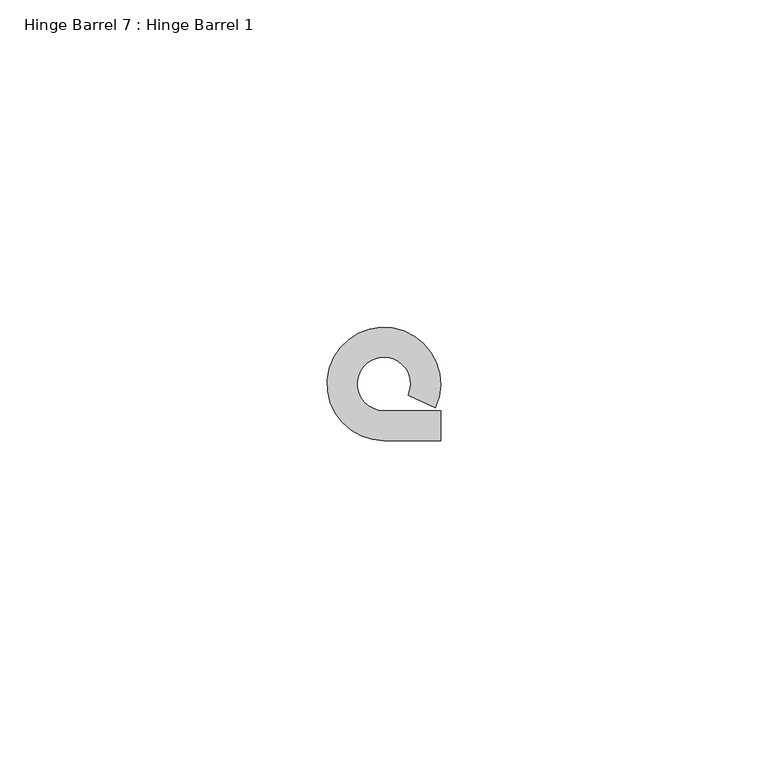
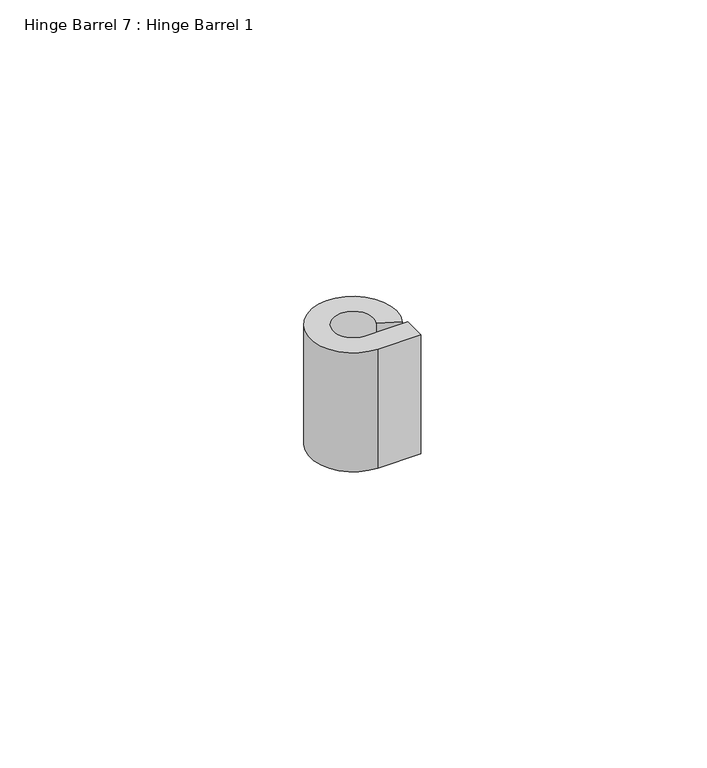
"""IFC4 building model written with IfcOpenShell, lengths in millimetres: proxy geometry, Hinge Barrel 7 : Hinge Barrel 1."""

import ifcopenshell
import ifcopenshell.guid

model = None  # the IFC model being written
_history = None  # IfcOwnerHistory: only IFC2X3 demands one
_inside = {}  # id of a spatial element -> (the spatial element, [elements in it])
_under = {}  # id of a project, library or spatial element -> (it, [spatial elements below it])
_declared = {}  # id of a project -> (the project, [libraries it declares])
_typed = {}  # id of a type object -> (the type object, [elements of that type])
_made_of = {}  # id of a material, layer set ... -> (it, [elements and type objects made of it])


def new_model(schema):
    """Start an empty IFC model of exactly this schema.

    Asked for "IFC4X3", IfcOpenShell would pick the latest addendum, in which some entities
    have other attributes; the version numbers below select the first issue.
    IFC2X3 requires an IfcOwnerHistory on every rooted entity: one is made here for all.
    """
    global model, _history
    if schema == "IFC4X3":
        model = ifcopenshell.file(schema_version=(4, 3, 0, 0))
    else:
        model = ifcopenshell.file(schema=schema)
    _inside.clear()
    _under.clear()
    _declared.clear()
    _typed.clear()
    _made_of.clear()
    _history = None
    if model.schema == "IFC2X3":
        org = make("IfcOrganization", Name="unknown")
        user = make(
            "IfcPersonAndOrganization",
            ThePerson=make("IfcPerson", FamilyName="unknown"),
            TheOrganization=org,
        )
        app = make(
            "IfcApplication",
            ApplicationDeveloper=org,
            Version="unknown",
            ApplicationFullName="unknown",
            ApplicationIdentifier="unknown",
        )
        _history = make(
            "IfcOwnerHistory",
            OwningUser=user,
            OwningApplication=app,
            ChangeAction="ADDED",
            CreationDate=0,
        )
    return model


def make(cls, **values):
    """One entity of the class cls with the attributes given. An attribute that is None is left unset."""
    return model.create_entity(
        cls, **{name: value for name, value in values.items() if value is not None}
    )


def rooted(cls, **values):
    """An entity with a GlobalId (a new one), such as an element, a storey or a relation."""
    return make(cls, GlobalId=ifcopenshell.guid.new(), OwnerHistory=_history, **values)


def si_unit(unit_type, name, prefix=None):
    """IfcSIUnit, for example si_unit("LENGTHUNIT", "METRE", prefix="MILLI")."""
    return make("IfcSIUnit", UnitType=unit_type, Prefix=prefix, Name=name)


def assignment(units):
    """IfcUnitAssignment: the units of a project."""
    return None if units is None else make("IfcUnitAssignment", Units=units)


def point(xyz):
    """IfcCartesianPoint."""
    return None if xyz is None else make("IfcCartesianPoint", Coordinates=xyz)


def direction(xyz):
    """IfcDirection."""
    return None if xyz is None else make("IfcDirection", DirectionRatios=xyz)


def frame(location, z_axis=None, x_axis=None):
    """IfcAxis2Placement3D, a coordinate frame: its origin and axes. An axis left out is left unset."""
    return make(
        "IfcAxis2Placement3D",
        Location=point(location),
        Axis=direction(z_axis),
        RefDirection=direction(x_axis),
    )


def frame_2d(location, x_axis=None):
    """IfcAxis2Placement2D, a coordinate frame in the plane: its origin and x axis."""
    return make(
        "IfcAxis2Placement2D", Location=point(location), RefDirection=direction(x_axis)
    )


def origin():
    """The frame at (0, 0, 0) with its axes left unset."""
    return frame((0.0, 0.0, 0.0))


def place(relative_to, where):
    """IfcLocalPlacement: puts the frame where relative to a parent placement (None: the world)."""
    return make(
        "IfcLocalPlacement", PlacementRelTo=relative_to, RelativePlacement=where
    )


def context(
    kind, dimensions, precision=None, world=None, true_north=None, identifier=None
):
    """IfcGeometricRepresentationContext, for example the 3D "Model" context."""
    return make(
        "IfcGeometricRepresentationContext",
        ContextIdentifier=identifier,
        ContextType=kind,
        CoordinateSpaceDimension=dimensions,
        Precision=precision,
        WorldCoordinateSystem=world,
        TrueNorth=true_north,
    )


def project(units=None, contexts=None):
    """IfcProject with its units and contexts."""
    return rooted(
        "IfcProject",
        Name="project",
        RepresentationContexts=contexts,
        UnitsInContext=assignment(units),
    )


def spatial(cls, under=None, at=None, **own):
    """A site, building, storey or space (cls), placed at a placement, below another one or the project."""
    s = rooted(cls, ObjectPlacement=at, **own)
    if under is not None:
        _under.setdefault(under.id(), (under, []))[1].append(s)
    return s


def polyline(points):
    """IfcPolyline through the points."""
    return make("IfcPolyline", Points=[point(p) for p in points])


def circle_curve(where, radius):
    """IfcCircle in the frame where."""
    return make("IfcCircle", Position=where, Radius=radius)


def trimmed(basis, trim1, trim2, sense, master):
    """IfcTrimmedCurve: the piece of a basis curve between two trims."""
    return make(
        "IfcTrimmedCurve",
        BasisCurve=basis,
        Trim1=trim1,
        Trim2=trim2,
        SenseAgreement=sense,
        MasterRepresentation=master,
    )


def segment(curve, same_sense, transition):
    """IfcCompositeCurveSegment."""
    return make(
        "IfcCompositeCurveSegment",
        Transition=transition,
        SameSense=same_sense,
        ParentCurve=curve,
    )


def composite_curve(segments, self_intersect=None):
    """IfcCompositeCurve: segments joined end to end."""
    return make("IfcCompositeCurve", Segments=segments, SelfIntersect=self_intersect)


def outline(outer, holes=None, kind="AREA"):
    """IfcArbitraryClosedProfileDef: a profile drawn as a closed curve; with holes, ...WithVoids."""
    if holes is None:
        return make("IfcArbitraryClosedProfileDef", ProfileType=kind, OuterCurve=outer)
    return make(
        "IfcArbitraryProfileDefWithVoids",
        ProfileType=kind,
        OuterCurve=outer,
        InnerCurves=holes,
    )


def extrude(swept, where, along, depth):
    """IfcExtrudedAreaSolid: the profile swept, set in the frame where, extruded along a direction by depth."""
    return make(
        "IfcExtrudedAreaSolid",
        SweptArea=swept,
        Position=where,
        ExtrudedDirection=direction(along),
        Depth=depth,
    )


def shape(context_of_items, identifier, shape_type, items):
    """IfcShapeRepresentation: the items that make up one representation, for example the "Body"."""
    return make(
        "IfcShapeRepresentation",
        ContextOfItems=context_of_items,
        RepresentationIdentifier=identifier,
        RepresentationType=shape_type,
        Items=items,
    )


def source(mapping_origin, context_of_items, identifier, shape_type, items):
    """IfcRepresentationMap: a shape defined once, which mapped items show again and again."""
    return make(
        "IfcRepresentationMap",
        MappingOrigin=mapping_origin,
        MappedRepresentation=shape(context_of_items, identifier, shape_type, items),
    )


def transform(
    local_origin,
    x_axis=None,
    y_axis=None,
    z_axis=None,
    scale=None,
    scale2=None,
    scale3=None,
    uniform=True,
):
    """IfcCartesianTransformationOperator3D, or its non-uniform kind. x_axis, y_axis, z_axis: its Axis1, 2, 3."""
    if uniform:
        return make(
            "IfcCartesianTransformationOperator3D",
            Axis1=direction(x_axis),
            Axis2=direction(y_axis),
            LocalOrigin=point(local_origin),
            Scale=scale,
            Axis3=direction(z_axis),
        )
    return make(
        "IfcCartesianTransformationOperator3DnonUniform",
        Axis1=direction(x_axis),
        Axis2=direction(y_axis),
        LocalOrigin=point(local_origin),
        Scale=scale,
        Axis3=direction(z_axis),
        Scale2=scale2,
        Scale3=scale3,
    )


def mapped(mapping_source, mapping_target):
    """IfcMappedItem: shows the shape of a source again, moved by a transform."""
    return make(
        "IfcMappedItem", MappingSource=mapping_source, MappingTarget=mapping_target
    )


def made_of(thing, what):
    """Note that an element or type object is made of a material, layer set ...; save() writes the relation."""
    if what is not None:
        _made_of.setdefault(what.id(), (what, []))[1].append(thing)
    return thing


def element(
    cls,
    number,
    at=None,
    inside=None,
    cuts=None,
    type_object=None,
    material=None,
    context=None,
    identifier="Body",
    shape_type=None,
    held_by="IfcProductDefinitionShape",
    body=None,
    shapes=None,
    **own,
):
    """One element of the class cls, such as IfcWall. Its Tag is "e" and its number.

    at: its placement. inside: the storey or other place that contains it. cuts: it is an
    opening in that element (IfcRelVoidsElement). A single representation is given by context,
    identifier, shape_type and body (its items); several are given by shapes. held_by: the class
    of the entity that holds the representations. save() writes the other relations.
    """
    e = rooted(cls, Tag="e%d" % number, ObjectPlacement=at, **own)
    if body is not None:
        shapes = [shape(context, identifier, shape_type, body)]
    if shapes is not None:
        e.Representation = make(held_by, Representations=shapes)
    if inside is not None:
        _inside.setdefault(inside.id(), (inside, []))[1].append(e)
    if cuts is not None:
        rooted(
            "IfcRelVoidsElement", RelatingBuildingElement=cuts, RelatedOpeningElement=e
        )
    if type_object is not None:
        _typed.setdefault(type_object.id(), (type_object, []))[1].append(e)
    return made_of(e, material)


def aggregate(whole, parts):
    """IfcRelAggregates: a whole, such as a stair, and the parts it consists of."""
    return rooted("IfcRelAggregates", RelatingObject=whole, RelatedObjects=parts)


def save(model, path):
    """Write the relations noted so far, then the file.

    IfcRelAggregates (storeys below a building ...), IfcRelContainedInSpatialStructure (elements
    in a storey), IfcRelDefinesByType, IfcRelAssociatesMaterial and IfcRelDeclares: one each for
    every whole, place, type object, material and project.
    """
    for whole, parts in _under.values():
        aggregate(whole, parts)
    for where, things in _inside.values():
        rooted(
            "IfcRelContainedInSpatialStructure",
            RelatedElements=things,
            RelatingStructure=where,
        )
    for kind, things in _typed.values():
        rooted("IfcRelDefinesByType", RelatedObjects=things, RelatingType=kind)
    for what, things in _made_of.values():
        rooted("IfcRelAssociatesMaterial", RelatedObjects=things, RelatingMaterial=what)
    for by, libraries in _declared.values():
        rooted("IfcRelDeclares", RelatingContext=by, RelatedDefinitions=libraries)
    model.write(path)


def hinge_barrel_7_hinge_barrel_1_4fbccd9d(model_context):
    return source(origin(), model_context, "Body", "SweptSolid", [
        extrude(outline(composite_curve([segment(polyline([(587323.2214739, -531780.6943841), (587327.7934739, -531780.6943841), (587327.7934739, -531785.2584466), (587319.1320739, -531785.2584466)]), True, "CONTINUOUS"), segment(trimmed(circle_curve(frame_2d((587319.1320739, -531776.6049841)), 8.6534625), [point((587319.1320739, -531785.2584466))], [point((587326.986084, -531780.2377433))], False, "CARTESIAN"), True, "CONTINUOUS"), segment(polyline([(587326.986084, -531780.2377433), (587322.8436736, -531778.321731)]), True, "CONTINUOUS"), segment(trimmed(circle_curve(frame_2d((587319.1320739, -531776.6049841)), 4.0894), [point((587322.8436736, -531778.321731))], [point((587319.1320739, -531780.6943841))], True, "CARTESIAN"), True, "CONTINUOUS"), segment(polyline([(587319.1320739, -531780.6943841), (587323.2214739, -531780.6943841)]), True, "CONTINUOUS")], self_intersect=False)), frame((0.0, 0.0, 1936.75), z_axis=(0.0, 0.0, 1.0), x_axis=(1.0, 0.0, 0.0)), (0.0, 0.0, 1.0), 25.4),
    ])


if __name__ == "__main__":
    model = new_model("IFC4")
    model_context = context("Model", 3, world=origin())
    ifc_project = project(units=[si_unit("LENGTHUNIT", "METRE", prefix="MILLI")], contexts=[model_context])
    site = spatial("IfcSite", under=ifc_project)
    building = spatial("IfcBuilding", under=site)
    placement = place(None, origin())
    hinge_barrel_7_hinge_barrel_1_shape = hinge_barrel_7_hinge_barrel_1_4fbccd9d(model_context)
    element("IfcBuildingElementProxy", 1, Name="Hinge Barrel 7 : Hinge Barrel 1", ObjectType="Hinge Barrel 7 : Hinge Barrel 1", at=placement, inside=building, context=model_context, shape_type="MappedRepresentation", body=[
        mapped(hinge_barrel_7_hinge_barrel_1_shape, transform((0.0, 0.0, 0.0), x_axis=(1.0, 0.0, 0.0), y_axis=(0.0, 1.0, 0.0), z_axis=(0.0, 0.0, 1.0))),
    ])
    save(model, "model.ifc")

# Revit data of these elements
# Element 1 (IfcBuildingElementProxy, "Hinge Barrel 7 : Hinge Barrel 1")
#   Materials on its faces: "6\"X6\" WELD-ON STL BUTT HINGE"
# Materials
#   "6\"X6\" WELD-ON STL BUTT HINGE": class "Metal", colour RGB 189 187 185, transparency 0, Description = "Carbon steel", Cost = 0
